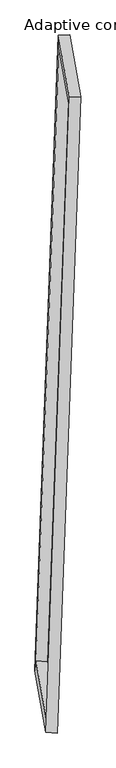
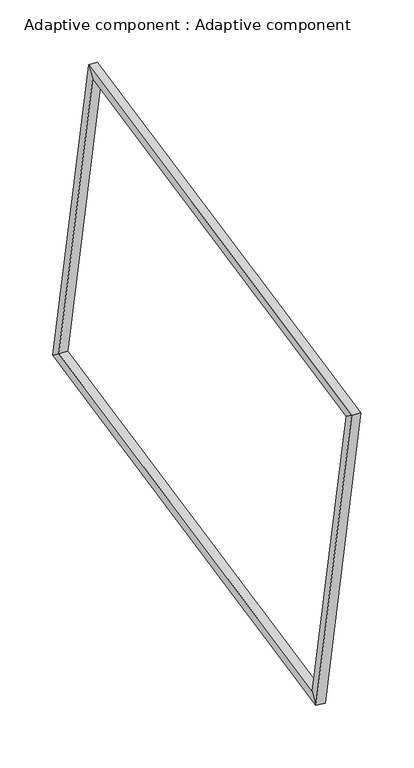
"""IFC4 building model written with IfcOpenShell, lengths in millimetres: proxy geometry, Adaptive component : Adaptive component."""

from ifc_helpers import new_model, si_unit, origin, place, context, project, spatial, faceted_brep, source, transform, mapped, element, save


def adaptive_component_adaptive_component_86ac6a02(model_context):
    return source(origin(), model_context, "Body", "Brep", [
        faceted_brep([(75.3336707, 1202.2276735, 2825.7856595), (140.362596, 1201.8043135, 2826.1186432), (78.4016411, 1550.723195, 369.980743), (13.4732271, 1550.5805486, 373.6320368), (73.3392986, 1147.0084196, 2752.3499376), (14.7231949, 1477.0915398, 428.8022455), (138.3682239, 1146.5850596, 2752.6829214), (79.6516089, 1477.2341862, 425.1509517), (-54.8637683, -2044.5024024, -137.3950203), (-119.6445299, -2040.6616935, -133.181576), (-113.6285873, -1985.5745427, -59.8660728), (-48.8478257, -1989.4152515, -64.0795171), (7.0971866, -2393.4212838, 2318.7428799), (-57.7840863, -2389.0145686, 2318.9720467), (-55.0124836, -2315.6576629, 2263.6816193), (9.8687893, -2320.064378, 2263.4524525)], [[[0, 1, 2, 3]], [[4, 0, 3, 5]], [[6, 4, 5, 7]], [[1, 6, 7, 2]], [[3, 2, 8, 9]], [[5, 3, 9, 10]], [[7, 5, 10, 11]], [[2, 7, 11, 8]], [[9, 8, 12, 13]], [[10, 9, 13, 14]], [[11, 10, 14, 15]], [[8, 11, 15, 12]], [[13, 12, 1, 0]], [[14, 13, 0, 4]], [[15, 14, 4, 6]], [[12, 15, 6, 1]]]),
    ])


if __name__ == "__main__":
    model = new_model("IFC4")
    model_context = context("Model", 3, world=origin())
    ifc_project = project(units=[si_unit("LENGTHUNIT", "METRE", prefix="MILLI")], contexts=[model_context])
    site = spatial("IfcSite", under=ifc_project)
    building = spatial("IfcBuilding", under=site)
    placement = place(None, origin())
    adaptive_component_adaptive_component_shape = adaptive_component_adaptive_component_86ac6a02(model_context)
    element("IfcBuildingElementProxy", 1, Name="Adaptive component : Adaptive component", ObjectType="Adaptive component : Adaptive component", at=placement, inside=building, context=model_context, shape_type="MappedRepresentation", body=[
        mapped(adaptive_component_adaptive_component_shape, transform((0.0, 0.0, 0.0), x_axis=(1.0, 0.0, 0.0), y_axis=(0.0, 1.0, 0.0), z_axis=(0.0, 0.0, 1.0))),
    ])
    save(model, "model.ifc")

# Revit data of these elements
# Type "Adaptive component : Adaptive component"
#   r [instance default] = 2063.125 mm
#   2r [instance default] = 4126.251 mm
#   Number [instance default] = 5
#   Default Elevation = 0
# Element 1 (IfcBuildingElementProxy, "Adaptive component : Adaptive component")
#   r = 2107.392 mm
#   2r = 4214.783 mm
#   Number = 6
